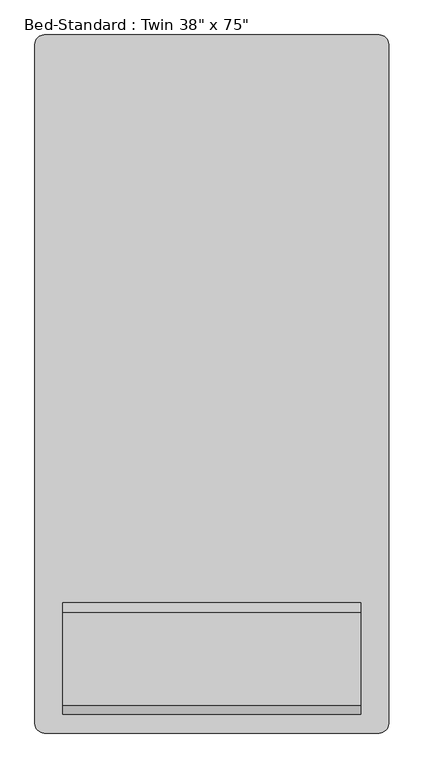
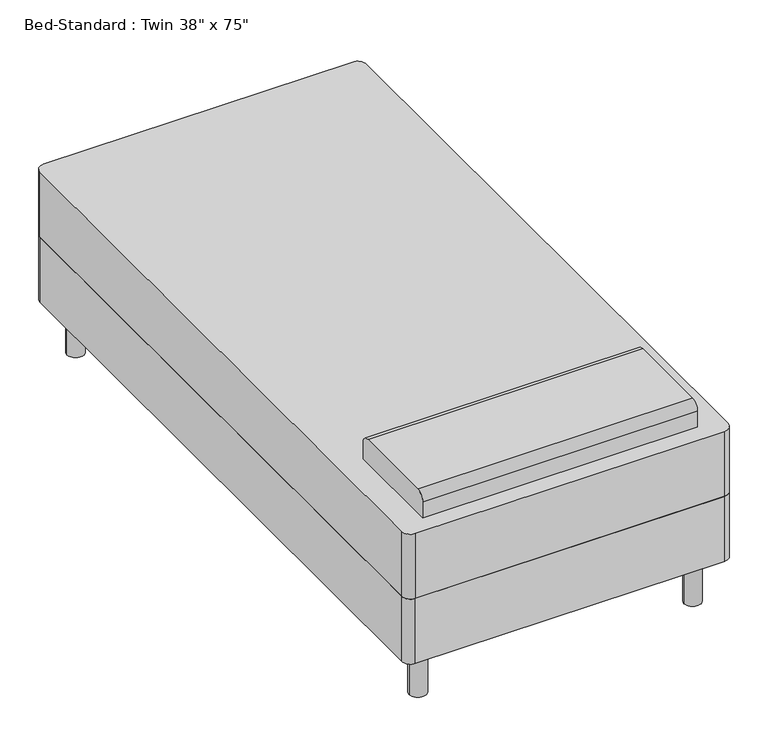
"""IFC4 building model written with IfcOpenShell, lengths in millimetres: furniture geometry."""

from ifc_helpers import new_model, si_unit, point, frame, frame_2d, origin, origin_with_axes, place, context, project, spatial, polyline, circle_curve, trimmed, segment, composite_curve, outline, extrude, source, transform, mapped, element, save


def furniture_89fb69ef(model_context):
    return source(origin(), model_context, "Body", "SweptSolid", [
        extrude(outline(composite_curve([segment(trimmed(circle_curve(frame_2d((-185.7114754, 972.695082)), 25.4), [point((-211.1114754, 972.695082))], [point((-185.7114754, 998.095082))], False, "CARTESIAN"), True, "CONTINUOUS"), segment(polyline([(-185.7114754, 998.095082), (728.6885246, 998.095082)]), True, "CONTINUOUS"), segment(trimmed(circle_curve(frame_2d((728.6885246, 972.695082)), 25.4), [point((728.6885246, 998.095082))], [point((754.0885246, 972.695082))], False, "CARTESIAN"), True, "CONTINUOUS"), segment(polyline([(754.0885246, 972.695082), (754.0885246, -881.504918)]), True, "CONTINUOUS"), segment(trimmed(circle_curve(frame_2d((728.6885246, -881.504918)), 25.4), [point((754.0885246, -881.504918))], [point((728.6885246, -906.904918))], False, "CARTESIAN"), True, "CONTINUOUS"), segment(polyline([(728.6885246, -906.904918), (-185.7114754, -906.904918)]), True, "CONTINUOUS"), segment(trimmed(circle_curve(frame_2d((-185.7114754, -881.504918)), 25.4), [point((-185.7114754, -906.904918))], [point((-211.1114754, -881.504918))], False, "CARTESIAN"), True, "CONTINUOUS"), segment(polyline([(-211.1114754, -881.504918), (-211.1114754, 972.695082)]), True, "CONTINUOUS")], self_intersect=False)), frame((0.0, 0.0, 152.4), z_axis=(0.0, 0.0, 1.0), x_axis=(1.0, 0.0, 0.0)), (0.0, 0.0, 1.0), 203.2),
        extrude(outline(composite_curve([segment(polyline([(-551.304918, 558.8), (-856.104918, 558.8), (-856.104918, 609.6)]), True, "CONTINUOUS"), segment(trimmed(circle_curve(frame_2d((-830.704918, 609.6)), 25.4), [point((-856.104918, 609.6))], [point((-830.704918, 635.0))], False, "CARTESIAN"), True, "CONTINUOUS"), segment(polyline([(-830.704918, 635.0), (-576.704918, 635.0)]), True, "CONTINUOUS"), segment(trimmed(circle_curve(frame_2d((-576.704918, 609.6)), 25.4), [point((-576.704918, 635.0))], [point((-551.304918, 609.6))], False, "CARTESIAN"), True, "CONTINUOUS"), segment(polyline([(-551.304918, 609.6), (-551.304918, 558.8)]), True, "CONTINUOUS")], self_intersect=False)), frame((-134.9114754, 0.0, 0.0), z_axis=(1.0, 0.0, 0.0), x_axis=(0.0, 1.0, 0.0)), (0.0, 0.0, 1.0), 812.8),
        extrude(outline(composite_curve([segment(trimmed(circle_curve(frame_2d((-134.9114754, -830.704918)), 25.4), [point((-160.3114754, -830.704918))], [point((-109.5114754, -830.704918))], False, "CARTESIAN"), True, "CONTINUOUS"), segment(trimmed(circle_curve(frame_2d((-134.9114754, -830.704918)), 25.4), [point((-109.5114754, -830.704918))], [point((-160.3114754, -830.704918))], False, "CARTESIAN"), True, "CONTINUOUS")], self_intersect=False)), origin_with_axes(), (0.0, 0.0, 1.0), 152.4),
        extrude(outline(composite_curve([segment(trimmed(circle_curve(frame_2d((677.8885246, -830.704918)), 25.4), [point((652.4885246, -830.704918))], [point((703.2885246, -830.704918))], False, "CARTESIAN"), True, "CONTINUOUS"), segment(trimmed(circle_curve(frame_2d((677.8885246, -830.704918)), 25.4), [point((703.2885246, -830.704918))], [point((652.4885246, -830.704918))], False, "CARTESIAN"), True, "CONTINUOUS")], self_intersect=False)), origin_with_axes(), (0.0, 0.0, 1.0), 152.4),
        extrude(outline(composite_curve([segment(trimmed(circle_curve(frame_2d((677.8885246, 921.895082)), 25.4), [point((652.4885246, 921.895082))], [point((703.2885246, 921.895082))], False, "CARTESIAN"), True, "CONTINUOUS"), segment(trimmed(circle_curve(frame_2d((677.8885246, 921.895082)), 25.4), [point((703.2885246, 921.895082))], [point((652.4885246, 921.895082))], False, "CARTESIAN"), True, "CONTINUOUS")], self_intersect=False)), origin_with_axes(), (0.0, 0.0, 1.0), 152.4),
        extrude(outline(composite_curve([segment(trimmed(circle_curve(frame_2d((-134.9114754, 921.895082)), 25.4), [point((-160.3114754, 921.895082))], [point((-109.5114754, 921.895082))], False, "CARTESIAN"), True, "CONTINUOUS"), segment(trimmed(circle_curve(frame_2d((-134.9114754, 921.895082)), 25.4), [point((-109.5114754, 921.895082))], [point((-160.3114754, 921.895082))], False, "CARTESIAN"), True, "CONTINUOUS")], self_intersect=False)), origin_with_axes(), (0.0, 0.0, 1.0), 152.4),
        extrude(outline(composite_curve([segment(trimmed(circle_curve(frame_2d((-185.7114754, -881.504918)), 25.4), [point((-185.7114754, -906.904918))], [point((-211.1114754, -881.504918))], False, "CARTESIAN"), True, "CONTINUOUS"), segment(polyline([(-211.1114754, -881.504918), (-211.1114754, 972.695082)]), True, "CONTINUOUS"), segment(trimmed(circle_curve(frame_2d((-185.7114754, 972.695082)), 25.4), [point((-211.1114754, 972.695082))], [point((-185.7114754, 998.095082))], False, "CARTESIAN"), True, "CONTINUOUS"), segment(polyline([(-185.7114754, 998.095082), (728.6885246, 998.095082)]), True, "CONTINUOUS"), segment(trimmed(circle_curve(frame_2d((728.6885246, 972.695082)), 25.4), [point((728.6885246, 998.095082))], [point((754.0885246, 972.695082))], False, "CARTESIAN"), True, "CONTINUOUS"), segment(polyline([(754.0885246, 972.695082), (754.0885246, -881.504918)]), True, "CONTINUOUS"), segment(trimmed(circle_curve(frame_2d((728.6885246, -881.504918)), 25.4), [point((754.0885246, -881.504918))], [point((728.6885246, -906.904918))], False, "CARTESIAN"), True, "CONTINUOUS"), segment(polyline([(728.6885246, -906.904918), (-185.7114754, -906.904918)]), True, "CONTINUOUS")], self_intersect=False)), frame((0.0, 0.0, 355.6), z_axis=(0.0, 0.0, 1.0), x_axis=(1.0, 0.0, 0.0)), (0.0, 0.0, 1.0), 203.2),
    ])


if __name__ == "__main__":
    model = new_model("IFC4")
    model_context = context("Model", 3, world=origin())
    ifc_project = project(units=[si_unit("LENGTHUNIT", "METRE", prefix="MILLI")], contexts=[model_context])
    site = spatial("IfcSite", under=ifc_project)
    building = spatial("IfcBuilding", under=site)
    placement = place(None, origin())
    furniture_shape = furniture_89fb69ef(model_context)
    element("IfcFurniture", 1, ObjectType="Bed-Standard : Twin 38\" x 75\"", at=placement, inside=building, context=model_context, shape_type="MappedRepresentation", body=[
        mapped(furniture_shape, transform((0.0, 0.0, 0.0), x_axis=(1.0, 0.0, 0.0), y_axis=(0.0, 1.0, 0.0), z_axis=(0.0, 0.0, 1.0))),
    ])
    save(model, "model.ifc")

# Revit data of these elements
# Type "Bed-Standard : Twin 38\" x 75\""
#   Assembly Code = "E2020200"
#   Clear Dim_2 = 2' - 0"
#   Clear Dim_1 = 3' - 0"
#   Length = 6' - 3"
#   Width = 3' - 2"
#   Leg Material = Metal - Chrome
#   Mattress Material = Textile - White
# Element 1 (IfcFurniture, "Bed-Standard : Twin 38\" x 75\"")
#   Materials on its faces: "Textile - White", "Metal - Chrome"
# Materials
#   "Metal - Chrome": class "Metal", colour RGB 17 17 17, transparency 0
#   "Textile - White": class "Fabric", colour RGB 247 247 239, transparency 0
